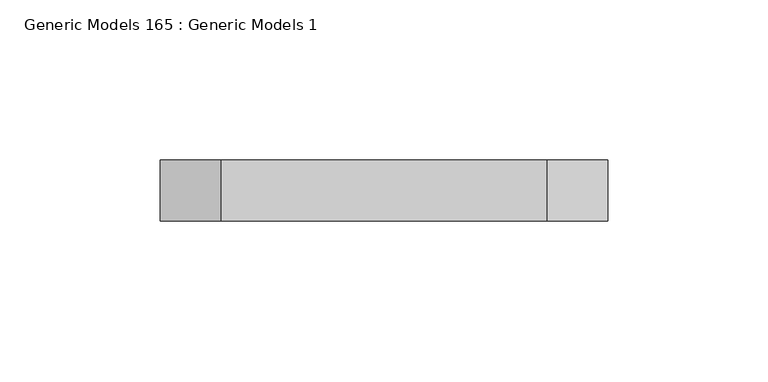
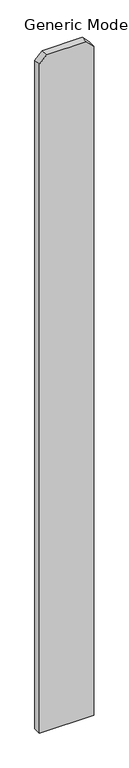
"""IFC4 building model written with IfcOpenShell, lengths in millimetres: proxy geometry, Generic Models 165 : Generic Models 1."""

from ifc_helpers import new_model, si_unit, frame, origin, place, context, project, spatial, polyline, outline, extrude, source, transform, mapped, element, save


def generic_models_165_generic_models_1_5969d6cb(model_context):
    return source(origin(), model_context, "Body", "SweptSolid", [
        extrude(outline(polyline([(76.2, 55141.8125), (1885.95, 55141.8125), (1905.0, 55122.7625), (1905.0, 55021.1625), (1885.95, 55002.1125), (76.2, 55002.1125), (76.2, 55141.8125)])), frame((0.0, 547.6875, 0.0), z_axis=(0.0, 1.0, 0.0), x_axis=(0.0, 0.0, 1.0)), (0.0, 0.0, 1.0), 19.05),
    ])


if __name__ == "__main__":
    model = new_model("IFC4")
    model_context = context("Model", 3, world=origin())
    ifc_project = project(units=[si_unit("LENGTHUNIT", "METRE", prefix="MILLI")], contexts=[model_context])
    site = spatial("IfcSite", under=ifc_project)
    building = spatial("IfcBuilding", under=site)
    placement = place(None, origin())
    generic_models_165_generic_models_1_shape = generic_models_165_generic_models_1_5969d6cb(model_context)
    element("IfcBuildingElementProxy", 1, Name="Generic Models 165 : Generic Models 1", ObjectType="Generic Models 165 : Generic Models 1", at=placement, inside=building, context=model_context, shape_type="MappedRepresentation", body=[
        mapped(generic_models_165_generic_models_1_shape, transform((0.0, 0.0, 0.0), x_axis=(1.0, 0.0, 0.0), y_axis=(0.0, 1.0, 0.0), z_axis=(0.0, 0.0, 1.0))),
    ])
    save(model, "model.ifc")

# Revit data of these elements
# Element 1 (IfcBuildingElementProxy, "Generic Models 165 : Generic Models 1")
#   Materials on its faces: "VERTICAL 1X6 CEDAR PLANKS W/ CLEAR WOOD SEALER"
# Materials
#   "VERTICAL 1X6 CEDAR PLANKS W/ CLEAR WOOD SEALER": class "Wood", colour RGB 234 198 147, transparency 0, Description = "Pinus Echinata", Cost = 0
